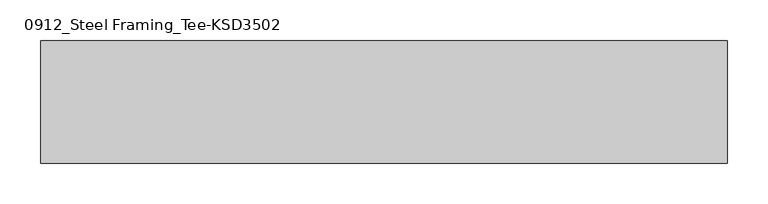
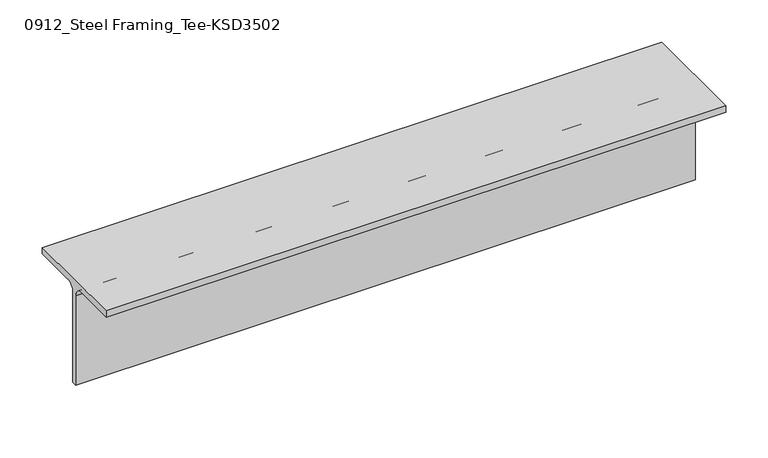
"""IFC4 building model written with IfcOpenShell, lengths in millimetres: member geometry, 0912_Steel Framing_Tee-KSD3502 : H_SB_ASB_CT-150x150x6.5x9."""

import ifcopenshell
import ifcopenshell.guid

model = None  # the IFC model being written
_history = None  # IfcOwnerHistory: only IFC2X3 demands one
_inside = {}  # id of a spatial element -> (the spatial element, [elements in it])
_under = {}  # id of a project, library or spatial element -> (it, [spatial elements below it])
_declared = {}  # id of a project -> (the project, [libraries it declares])
_typed = {}  # id of a type object -> (the type object, [elements of that type])
_made_of = {}  # id of a material, layer set ... -> (it, [elements and type objects made of it])


def new_model(schema):
    """Start an empty IFC model of exactly this schema.

    Asked for "IFC4X3", IfcOpenShell would pick the latest addendum, in which some entities
    have other attributes; the version numbers below select the first issue.
    IFC2X3 requires an IfcOwnerHistory on every rooted entity: one is made here for all.
    """
    global model, _history
    if schema == "IFC4X3":
        model = ifcopenshell.file(schema_version=(4, 3, 0, 0))
    else:
        model = ifcopenshell.file(schema=schema)
    _inside.clear()
    _under.clear()
    _declared.clear()
    _typed.clear()
    _made_of.clear()
    _history = None
    if model.schema == "IFC2X3":
        org = make("IfcOrganization", Name="unknown")
        user = make(
            "IfcPersonAndOrganization",
            ThePerson=make("IfcPerson", FamilyName="unknown"),
            TheOrganization=org,
        )
        app = make(
            "IfcApplication",
            ApplicationDeveloper=org,
            Version="unknown",
            ApplicationFullName="unknown",
            ApplicationIdentifier="unknown",
        )
        _history = make(
            "IfcOwnerHistory",
            OwningUser=user,
            OwningApplication=app,
            ChangeAction="ADDED",
            CreationDate=0,
        )
    return model


def make(cls, **values):
    """One entity of the class cls with the attributes given. An attribute that is None is left unset."""
    return model.create_entity(
        cls, **{name: value for name, value in values.items() if value is not None}
    )


def rooted(cls, **values):
    """An entity with a GlobalId (a new one), such as an element, a storey or a relation."""
    return make(cls, GlobalId=ifcopenshell.guid.new(), OwnerHistory=_history, **values)


def si_unit(unit_type, name, prefix=None):
    """IfcSIUnit, for example si_unit("LENGTHUNIT", "METRE", prefix="MILLI")."""
    return make("IfcSIUnit", UnitType=unit_type, Prefix=prefix, Name=name)


def assignment(units):
    """IfcUnitAssignment: the units of a project."""
    return None if units is None else make("IfcUnitAssignment", Units=units)


def point(xyz):
    """IfcCartesianPoint."""
    return None if xyz is None else make("IfcCartesianPoint", Coordinates=xyz)


def direction(xyz):
    """IfcDirection."""
    return None if xyz is None else make("IfcDirection", DirectionRatios=xyz)


def frame(location, z_axis=None, x_axis=None):
    """IfcAxis2Placement3D, a coordinate frame: its origin and axes. An axis left out is left unset."""
    return make(
        "IfcAxis2Placement3D",
        Location=point(location),
        Axis=direction(z_axis),
        RefDirection=direction(x_axis),
    )


def frame_2d(location, x_axis=None):
    """IfcAxis2Placement2D, a coordinate frame in the plane: its origin and x axis."""
    return make(
        "IfcAxis2Placement2D", Location=point(location), RefDirection=direction(x_axis)
    )


def origin():
    """The frame at (0, 0, 0) with its axes left unset."""
    return frame((0.0, 0.0, 0.0))


def place(relative_to, where):
    """IfcLocalPlacement: puts the frame where relative to a parent placement (None: the world)."""
    return make(
        "IfcLocalPlacement", PlacementRelTo=relative_to, RelativePlacement=where
    )


def context(
    kind, dimensions, precision=None, world=None, true_north=None, identifier=None
):
    """IfcGeometricRepresentationContext, for example the 3D "Model" context."""
    return make(
        "IfcGeometricRepresentationContext",
        ContextIdentifier=identifier,
        ContextType=kind,
        CoordinateSpaceDimension=dimensions,
        Precision=precision,
        WorldCoordinateSystem=world,
        TrueNorth=true_north,
    )


def project(units=None, contexts=None):
    """IfcProject with its units and contexts."""
    return rooted(
        "IfcProject",
        Name="project",
        RepresentationContexts=contexts,
        UnitsInContext=assignment(units),
    )


def spatial(cls, under=None, at=None, **own):
    """A site, building, storey or space (cls), placed at a placement, below another one or the project."""
    s = rooted(cls, ObjectPlacement=at, **own)
    if under is not None:
        _under.setdefault(under.id(), (under, []))[1].append(s)
    return s


def polyline(points):
    """IfcPolyline through the points."""
    return make("IfcPolyline", Points=[point(p) for p in points])


def circle_curve(where, radius):
    """IfcCircle in the frame where."""
    return make("IfcCircle", Position=where, Radius=radius)


def trimmed(basis, trim1, trim2, sense, master):
    """IfcTrimmedCurve: the piece of a basis curve between two trims."""
    return make(
        "IfcTrimmedCurve",
        BasisCurve=basis,
        Trim1=trim1,
        Trim2=trim2,
        SenseAgreement=sense,
        MasterRepresentation=master,
    )


def segment(curve, same_sense, transition):
    """IfcCompositeCurveSegment."""
    return make(
        "IfcCompositeCurveSegment",
        Transition=transition,
        SameSense=same_sense,
        ParentCurve=curve,
    )


def composite_curve(segments, self_intersect=None):
    """IfcCompositeCurve: segments joined end to end."""
    return make("IfcCompositeCurve", Segments=segments, SelfIntersect=self_intersect)


def outline(outer, holes=None, kind="AREA"):
    """IfcArbitraryClosedProfileDef: a profile drawn as a closed curve; with holes, ...WithVoids."""
    if holes is None:
        return make("IfcArbitraryClosedProfileDef", ProfileType=kind, OuterCurve=outer)
    return make(
        "IfcArbitraryProfileDefWithVoids",
        ProfileType=kind,
        OuterCurve=outer,
        InnerCurves=holes,
    )


def extrude(swept, where, along, depth):
    """IfcExtrudedAreaSolid: the profile swept, set in the frame where, extruded along a direction by depth."""
    return make(
        "IfcExtrudedAreaSolid",
        SweptArea=swept,
        Position=where,
        ExtrudedDirection=direction(along),
        Depth=depth,
    )


def shape(context_of_items, identifier, shape_type, items):
    """IfcShapeRepresentation: the items that make up one representation, for example the "Body"."""
    return make(
        "IfcShapeRepresentation",
        ContextOfItems=context_of_items,
        RepresentationIdentifier=identifier,
        RepresentationType=shape_type,
        Items=items,
    )


def source(mapping_origin, context_of_items, identifier, shape_type, items):
    """IfcRepresentationMap: a shape defined once, which mapped items show again and again."""
    return make(
        "IfcRepresentationMap",
        MappingOrigin=mapping_origin,
        MappedRepresentation=shape(context_of_items, identifier, shape_type, items),
    )


def transform(
    local_origin,
    x_axis=None,
    y_axis=None,
    z_axis=None,
    scale=None,
    scale2=None,
    scale3=None,
    uniform=True,
):
    """IfcCartesianTransformationOperator3D, or its non-uniform kind. x_axis, y_axis, z_axis: its Axis1, 2, 3."""
    if uniform:
        return make(
            "IfcCartesianTransformationOperator3D",
            Axis1=direction(x_axis),
            Axis2=direction(y_axis),
            LocalOrigin=point(local_origin),
            Scale=scale,
            Axis3=direction(z_axis),
        )
    return make(
        "IfcCartesianTransformationOperator3DnonUniform",
        Axis1=direction(x_axis),
        Axis2=direction(y_axis),
        LocalOrigin=point(local_origin),
        Scale=scale,
        Axis3=direction(z_axis),
        Scale2=scale2,
        Scale3=scale3,
    )


def mapped(mapping_source, mapping_target):
    """IfcMappedItem: shows the shape of a source again, moved by a transform."""
    return make(
        "IfcMappedItem", MappingSource=mapping_source, MappingTarget=mapping_target
    )


def made_of(thing, what):
    """Note that an element or type object is made of a material, layer set ...; save() writes the relation."""
    if what is not None:
        _made_of.setdefault(what.id(), (what, []))[1].append(thing)
    return thing


def element(
    cls,
    number,
    at=None,
    inside=None,
    cuts=None,
    type_object=None,
    material=None,
    context=None,
    identifier="Body",
    shape_type=None,
    held_by="IfcProductDefinitionShape",
    body=None,
    shapes=None,
    **own,
):
    """One element of the class cls, such as IfcWall. Its Tag is "e" and its number.

    at: its placement. inside: the storey or other place that contains it. cuts: it is an
    opening in that element (IfcRelVoidsElement). A single representation is given by context,
    identifier, shape_type and body (its items); several are given by shapes. held_by: the class
    of the entity that holds the representations. save() writes the other relations.
    """
    e = rooted(cls, Tag="e%d" % number, ObjectPlacement=at, **own)
    if body is not None:
        shapes = [shape(context, identifier, shape_type, body)]
    if shapes is not None:
        e.Representation = make(held_by, Representations=shapes)
    if inside is not None:
        _inside.setdefault(inside.id(), (inside, []))[1].append(e)
    if cuts is not None:
        rooted(
            "IfcRelVoidsElement", RelatingBuildingElement=cuts, RelatedOpeningElement=e
        )
    if type_object is not None:
        _typed.setdefault(type_object.id(), (type_object, []))[1].append(e)
    return made_of(e, material)


def aggregate(whole, parts):
    """IfcRelAggregates: a whole, such as a stair, and the parts it consists of."""
    return rooted("IfcRelAggregates", RelatingObject=whole, RelatedObjects=parts)


def save(model, path):
    """Write the relations noted so far, then the file.

    IfcRelAggregates (storeys below a building ...), IfcRelContainedInSpatialStructure (elements
    in a storey), IfcRelDefinesByType, IfcRelAssociatesMaterial and IfcRelDeclares: one each for
    every whole, place, type object, material and project.
    """
    for whole, parts in _under.values():
        aggregate(whole, parts)
    for where, things in _inside.values():
        rooted(
            "IfcRelContainedInSpatialStructure",
            RelatedElements=things,
            RelatingStructure=where,
        )
    for kind, things in _typed.values():
        rooted("IfcRelDefinesByType", RelatedObjects=things, RelatingType=kind)
    for what, things in _made_of.values():
        rooted("IfcRelAssociatesMaterial", RelatedObjects=things, RelatingMaterial=what)
    for by, libraries in _declared.values():
        rooted("IfcRelDeclares", RelatingContext=by, RelatedDefinitions=libraries)
    model.write(path)


def member_0912_steel_framing_tee_ksd3502_7caef576(model_context):
    return source(origin(), model_context, "Body", "SweptSolid", [
        extrude(outline(composite_curve([segment(polyline([(-75.0, 75.0), (75.0, 75.0), (75.0, 66.0), (16.25, 66.0)]), True, "CONTINUOUS"), segment(trimmed(circle_curve(frame_2d((16.25, 53.0)), 13.0), [point((16.25, 66.0))], [point((3.25, 53.0))], True, "CARTESIAN"), True, "CONTINUOUS"), segment(polyline([(3.25, 53.0), (3.25, -75.0), (-3.25, -75.0), (-3.25, 53.0)]), True, "CONTINUOUS"), segment(trimmed(circle_curve(frame_2d((-16.25, 53.0)), 13.0), [point((-3.25, 53.0))], [point((-16.25, 66.0))], True, "CARTESIAN"), True, "CONTINUOUS"), segment(polyline([(-16.25, 66.0), (-75.0, 66.0), (-75.0, 75.0)]), True, "CONTINUOUS")], self_intersect=False)), frame((-500.0, 0.0, 0.0), z_axis=(1.0, 0.0, 0.0), x_axis=(0.0, 1.0, 0.0)), (0.0, 0.0, 1.0), 841.5),
    ])


if __name__ == "__main__":
    model = new_model("IFC4")
    model_context = context("Model", 3, world=origin())
    ifc_project = project(units=[si_unit("LENGTHUNIT", "METRE", prefix="MILLI")], contexts=[model_context])
    site = spatial("IfcSite", under=ifc_project)
    building = spatial("IfcBuilding", under=site)
    placement = place(None, origin())
    member_0912_steel_framing_tee_ksd3502_shape = member_0912_steel_framing_tee_ksd3502_7caef576(model_context)
    element("IfcMember", 1, ObjectType="0912_Steel Framing_Tee-KSD3502 : H_SB_ASB_CT-150x150x6.5x9", at=placement, inside=building, context=model_context, shape_type="MappedRepresentation", body=[
        mapped(member_0912_steel_framing_tee_ksd3502_shape, transform((0.0, 0.0, 0.0), x_axis=(1.0, 0.0, 0.0), y_axis=(0.0, 1.0, 0.0), z_axis=(0.0, 0.0, 1.0))),
    ])
    save(model, "model.ifc")

# Revit data of these elements
# Type "0912_Steel Framing_Tee-KSD3502 : H_SB_ASB_CT-150x150x6.5x9"
#   H_WM Code_1 = "S01AA003-00001 | Main Steel Structure Fabrication Work | Shelter/Building | Light Steel - Standard (30KG/M>Weight) | Material: (   )"
#   H_WM Code_2 = "S03AA029-00001 | Main Steel Structure Erection Work | Shelter/Building | Light Steel (30KG/M>Weight) | Material: (   )"
#   H_WM Code_3 = "S01AA010-00001 | Main Steel Structure Fabrication Work | Shelter/Building | Steel Painting/Coating | for Non-Fireproofed Steel Surface, Surface Preparation, Primer, Second & Final Coat | Material: (   )"
#   H_Q'ty Cal Type Tag = "SB-Q2"
#   Width = 15.0 cm
#   Web Thickness = 0.65 cm
#   Web Fillet = 1.3 cm
#   Section Area = 23.39 cm²
#   Perimeter = 0.60 m²/m
#   Nominal Weight = 18.40 kgf/m
#   Height = 15.0 cm
#   Flange Thickness = 0.9 cm
#   Centroid Vertical = 7.5 cm
#   Centroid Horizontal = 7.5 cm
#   Length [instance default] = 1.5000 m
#   Structural Material [instance default] = Steel, 45-345
#   Warping Constant = (empty or 0)
#   Torsional Moment of Inertia = 0
#   Section Name Key = ""
#   Plastic Modulus weak axis = 0
#   Plastic Modulus strong axis = 0
#   Moment of Inertia weak axis = 0
#   Moment of Inertia strong axis = 0
#   Elastic Modulus weak axis = 0
#   Elastic Modulus strong axis = 0
#   Bolt Spacing = 0
#   Assembly Code = ""
# Element 1 (IfcMember, "0912_Steel Framing_Tee-KSD3502 : H_SB_ASB_CT-150x150x6.5x9")
#   Structural Material = none
# Materials
#   "Steel, 45-345": class "Metal", colour RGB 189 187 185, transparency 0, Description = "Steel 345 MPa", Cost = 0
